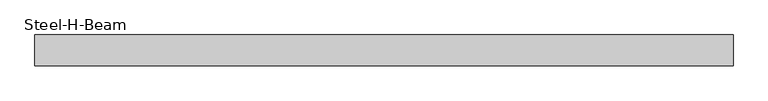
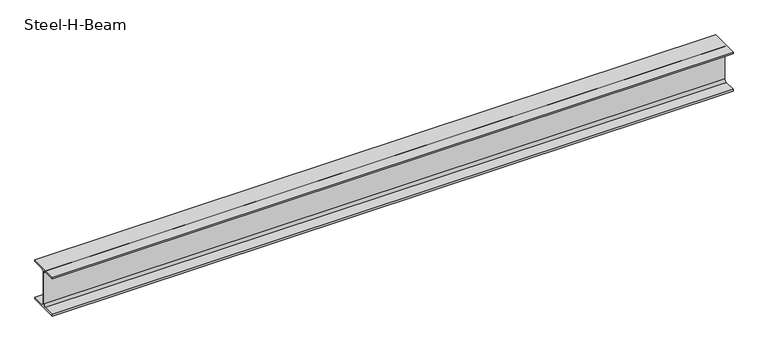
"""IFC4 building model written with IfcOpenShell, lengths in millimetres: beam geometry, Steel-H-Beam : BM121_H-340×250x9x14."""

from ifc_helpers import new_model, si_unit, point, frame, frame_2d, origin, place, context, project, spatial, polyline, circle_curve, trimmed, segment, composite_curve, outline, extrude, source, transform, mapped, element, save


def steel_h_beam_dded6d60(model_context):
    return source(origin(), model_context, "Body", "SweptSolid", [
        extrude(outline(composite_curve([segment(polyline([(125.0, -156.0), (125.0, -170.0), (-125.0, -170.0), (-125.0, -156.0), (-24.5, -156.0)]), True, "CONTINUOUS"), segment(trimmed(circle_curve(frame_2d((-24.5, -136.0)), 20.0), [point((-24.5, -156.0))], [point((-4.5, -136.0))], True, "CARTESIAN"), True, "CONTINUOUS"), segment(polyline([(-4.5, -136.0), (-4.5, 136.0)]), True, "CONTINUOUS"), segment(trimmed(circle_curve(frame_2d((-24.5, 136.0)), 20.0), [point((-4.5, 136.0))], [point((-24.5, 156.0))], True, "CARTESIAN"), True, "CONTINUOUS"), segment(polyline([(-24.5, 156.0), (-125.0, 156.0), (-125.0, 170.0), (125.0, 170.0), (125.0, 156.0), (24.5, 156.0)]), True, "CONTINUOUS"), segment(trimmed(circle_curve(frame_2d((24.5, 136.0)), 20.0), [point((24.5, 156.0))], [point((4.5, 136.0))], True, "CARTESIAN"), True, "CONTINUOUS"), segment(polyline([(4.5, 136.0), (4.5, -136.0)]), True, "CONTINUOUS"), segment(trimmed(circle_curve(frame_2d((24.5, -136.0)), 20.0), [point((4.5, -136.0))], [point((24.5, -156.0))], True, "CARTESIAN"), True, "CONTINUOUS"), segment(polyline([(24.5, -156.0), (125.0, -156.0)]), True, "CONTINUOUS")], self_intersect=False)), frame((-2854.7871653, 0.0, 0.0), z_axis=(1.0, 0.0, 0.0), x_axis=(0.0, 1.0, 0.0)), (0.0, 0.0, 1.0), 5636.1638128),
    ])


if __name__ == "__main__":
    model = new_model("IFC4")
    model_context = context("Model", 3, world=origin())
    ifc_project = project(units=[si_unit("LENGTHUNIT", "METRE", prefix="MILLI")], contexts=[model_context])
    site = spatial("IfcSite", under=ifc_project)
    building = spatial("IfcBuilding", under=site)
    placement = place(None, origin())
    steel_h_beam_shape = steel_h_beam_dded6d60(model_context)
    element("IfcBeam", 1, ObjectType="Steel-H-Beam : BM121_H-340×250x9x14", at=placement, inside=building, context=model_context, shape_type="MappedRepresentation", body=[
        mapped(steel_h_beam_shape, transform((0.0, 0.0, 0.0), x_axis=(1.0, 0.0, 0.0), y_axis=(0.0, 1.0, 0.0), z_axis=(0.0, 0.0, 1.0))),
    ])
    save(model, "model.ifc")

# Revit data of these elements
# Type "Steel-H-Beam : BM121_H-340×250x9x14"
#   Surface Area = 1.62766 m²/m
#   Section Area = 101.514 cm²
#   Mass per Unit Length = 79.6882 kg/m
#   Length [instance default] = 3000 mm
#   B = 250 mm
#   H = 340 mm
#   r = 20 mm
#   tw = 9 mm
#   tf = 14 mm
#   hec_material4 [instance default] = none
#   hec_material3 [instance default] = none
#   hec_material2 [instance default] = none
#   hec_material1 [instance default] = none
#   Structural Material [instance default] = Steel, 45-345
#   Assembly Code = ""
# Element 1 (IfcBeam, "Steel-H-Beam : BM121_H-340×250x9x14")
#   hec_material4 = S01AA010-00002_Main Steel Structure Fabrication Work_Shelter/Building_Steel Painting/Coating_for Fireproofed Steel Surface, Surface Preparation & Primer Coat
#   hec_material3 = F01AC000-00002_Building/Shelter Fire Proofing Work_Intumescent Coating Type_1 hr. rating (UL 1709))
#   hec_material2 = S01AA010-00002_Main Steel Structure Fabrication Work_Shelter/Building_Steel Painting/Coating_for Fireproofed Steel Surface, Surface Preparation & Primer Coat
#   hec_material1 = S03AA028-00001_Main Steel Structure Erection Work_Shelter/Building_Medium Steel
#   Structural Material = S01AA002-00001_Main Steel Structure Fabrication Work_Shelter/Building_Medium Steel - Standard
#   Materials on its faces: "S01AA002-00001_Main Steel Structure Fabrication Work_Shelter/Building_Medium Steel - Standard"
# Materials
#   "Steel, 45-345": class "Metal", colour RGB 189 187 185, transparency 0, Description = "Steel 345 MPa", Cost = 0
#   "S01AA002-00001_Main Steel Structure Fabrication Work_Shelter/Building_Medium Steel - Standard": class "Metal", colour RGB 120 120 120, transparency 0, Comments = "(90KG/M>Weight≥30KG/M)", Description = "Structural steel 50ksi", W00) Work Master Code = "S01AA002-0001", W01) Work Master_Lv1 = "Main Steel Structure Fabrication Work", W02) Work Master_Lv2 = "Shelter/Building", W03) Work Master_Spec.1 = "Medium Steel - Standard (90KG/M>Weight≥30KG/M)", Cost = 0
#   "S01AA010-00002_Main Steel Structure Fabrication Work_Shelter/Building_Steel Painting/Coating_for Fireproofed Steel Surface, Surface Preparation & Primer Coat": class "Metal", colour RGB 120 120 120, transparency 0, Description = "Paint finished steel", W00) Work Master Code = "SS01AA010-00002", W01) Work Master_Lv1 = "Main Steel Structure Fabrication Work", W02) Work Master_Lv2 = "Shelter/Building", W03) Work Master_Spec.1 = "Steel Painting/Coating", W04) Work Master_Spec.2 = "for Fireproofed Steel Surface, Surface Preparation & Primer Coat", Cost = 0
#   "F01AC000-00002_Building/Shelter Fire Proofing Work_Intumescent Coating Type_1 hr. rating (UL 1709))": class "Metal", colour RGB 255 128 128, transparency 0, Description = "Paint finished steel", W00) Work Master Code = "F01AC000-00002", W01) Work Master_Lv1 = "Building/Shelter Fire Proofing Work", W02) Work Master_Lv2 = "Intumescent Coating Type", W03) Work Master_Spec.1 = "1 hr. rating (UL 1709)", Cost = 0
#   "S03AA028-00001_Main Steel Structure Erection Work_Shelter/Building_Medium Steel": class "Metal", colour RGB 120 120 120, transparency 0, Comments = "(90KG/M>Weight≥30KG/M)", Description = "Structural steel 50ksi", W00) Work Master Code = "S03AA028-0001", W01) Work Master_Lv1 = "Main Steel Structure Erection Work", W02) Work Master_Lv2 = "Shelter/Building", W03) Work Master_Spec.1 = "Medium Steel (90KG/M>Weight≥30KG/M)", Cost = 0
